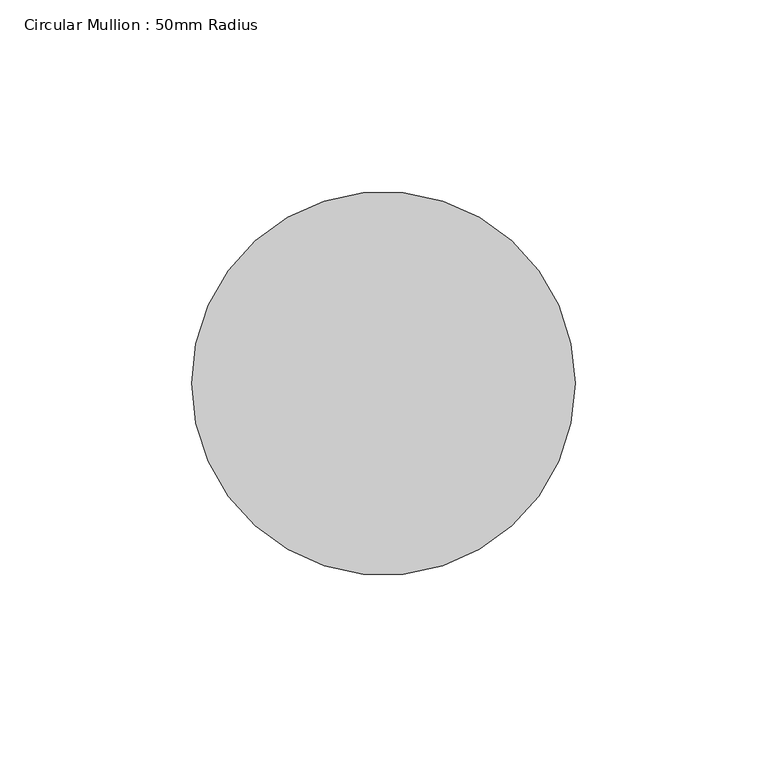
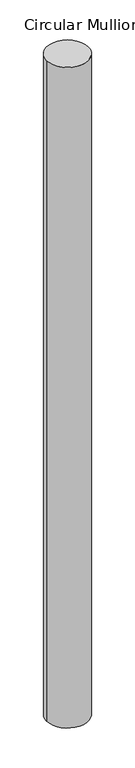
"""IFC4 building model written with IfcOpenShell, lengths in millimetres: member geometry, Circular Mullion : 50mm Radius."""

from ifc_helpers import new_model, si_unit, point, frame, origin, origin_2d, place, context, project, spatial, circle_curve, trimmed, segment, composite_curve, outline, extrude, source, transform, mapped, element, save


def circular_mullion_50mm_radius_805578a4(model_context):
    return source(origin(), model_context, "Body", "SweptSolid", [
        extrude(outline(composite_curve([segment(trimmed(circle_curve(origin_2d(), 50.0), [point((50.0, 0.0))], [point((-50.0, 0.0))], False, "CARTESIAN"), True, "CONTINUOUS"), segment(trimmed(circle_curve(origin_2d(), 50.0), [point((-50.0, 0.0))], [point((50.0, 0.0))], False, "CARTESIAN"), True, "CONTINUOUS")], self_intersect=False)), frame((0.0, 0.0, -1680.089134), z_axis=(0.0, 0.0, 1.0), x_axis=(1.0, 0.0, 0.0)), (0.0, 0.0, 1.0), 1680.089134),
    ])


if __name__ == "__main__":
    model = new_model("IFC4")
    model_context = context("Model", 3, world=origin())
    ifc_project = project(units=[si_unit("LENGTHUNIT", "METRE", prefix="MILLI")], contexts=[model_context])
    site = spatial("IfcSite", under=ifc_project)
    building = spatial("IfcBuilding", under=site)
    placement = place(None, origin())
    circular_mullion_50mm_radius_shape = circular_mullion_50mm_radius_805578a4(model_context)
    element("IfcMember", 1, ObjectType="Circular Mullion : 50mm Radius", at=placement, inside=building, context=model_context, shape_type="MappedRepresentation", body=[
        mapped(circular_mullion_50mm_radius_shape, transform((0.0, 0.0, 0.0), x_axis=(1.0, 0.0, 0.0), y_axis=(0.0, 1.0, 0.0), z_axis=(0.0, 0.0, 1.0))),
    ])
    save(model, "model.ifc")

# Revit data of these elements
# Type "Circular Mullion : 50mm Radius"
#   built-in parameter 1007350 = 0.164042 (stored number, unit not read)
# Element 1 (IfcMember, "Circular Mullion : 50mm Radius")
#   Materials on its faces: "Aluminium"
# Materials
#   "Aluminium": class "Metal", colour RGB 247 247 247, transparency 0, Description = "Aluminium 6061", Cost = 0
